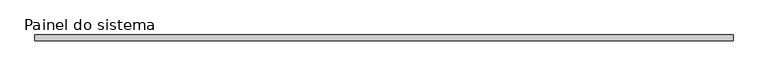
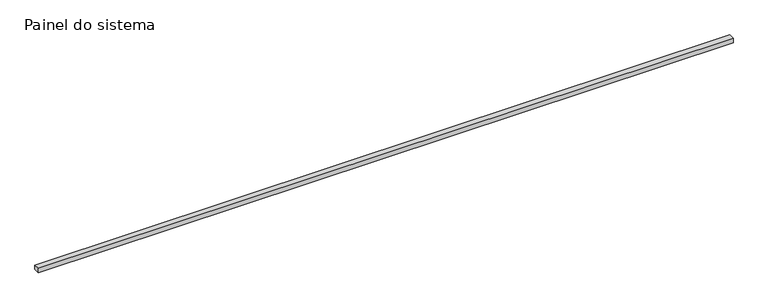
"""IFC4 building model written with IfcOpenShell, lengths in millimetres: plate geometry, Painel do sistema : Envidraçado."""

import ifcopenshell
import ifcopenshell.guid

model = None  # the IFC model being written
_history = None  # IfcOwnerHistory: only IFC2X3 demands one
_inside = {}  # id of a spatial element -> (the spatial element, [elements in it])
_under = {}  # id of a project, library or spatial element -> (it, [spatial elements below it])
_declared = {}  # id of a project -> (the project, [libraries it declares])
_typed = {}  # id of a type object -> (the type object, [elements of that type])
_made_of = {}  # id of a material, layer set ... -> (it, [elements and type objects made of it])


def new_model(schema):
    """Start an empty IFC model of exactly this schema.

    Asked for "IFC4X3", IfcOpenShell would pick the latest addendum, in which some entities
    have other attributes; the version numbers below select the first issue.
    IFC2X3 requires an IfcOwnerHistory on every rooted entity: one is made here for all.
    """
    global model, _history
    if schema == "IFC4X3":
        model = ifcopenshell.file(schema_version=(4, 3, 0, 0))
    else:
        model = ifcopenshell.file(schema=schema)
    _inside.clear()
    _under.clear()
    _declared.clear()
    _typed.clear()
    _made_of.clear()
    _history = None
    if model.schema == "IFC2X3":
        org = make("IfcOrganization", Name="unknown")
        user = make(
            "IfcPersonAndOrganization",
            ThePerson=make("IfcPerson", FamilyName="unknown"),
            TheOrganization=org,
        )
        app = make(
            "IfcApplication",
            ApplicationDeveloper=org,
            Version="unknown",
            ApplicationFullName="unknown",
            ApplicationIdentifier="unknown",
        )
        _history = make(
            "IfcOwnerHistory",
            OwningUser=user,
            OwningApplication=app,
            ChangeAction="ADDED",
            CreationDate=0,
        )
    return model


def make(cls, **values):
    """One entity of the class cls with the attributes given. An attribute that is None is left unset."""
    return model.create_entity(
        cls, **{name: value for name, value in values.items() if value is not None}
    )


def rooted(cls, **values):
    """An entity with a GlobalId (a new one), such as an element, a storey or a relation."""
    return make(cls, GlobalId=ifcopenshell.guid.new(), OwnerHistory=_history, **values)


def si_unit(unit_type, name, prefix=None):
    """IfcSIUnit, for example si_unit("LENGTHUNIT", "METRE", prefix="MILLI")."""
    return make("IfcSIUnit", UnitType=unit_type, Prefix=prefix, Name=name)


def assignment(units):
    """IfcUnitAssignment: the units of a project."""
    return None if units is None else make("IfcUnitAssignment", Units=units)


def point(xyz):
    """IfcCartesianPoint."""
    return None if xyz is None else make("IfcCartesianPoint", Coordinates=xyz)


def direction(xyz):
    """IfcDirection."""
    return None if xyz is None else make("IfcDirection", DirectionRatios=xyz)


def frame(location, z_axis=None, x_axis=None):
    """IfcAxis2Placement3D, a coordinate frame: its origin and axes. An axis left out is left unset."""
    return make(
        "IfcAxis2Placement3D",
        Location=point(location),
        Axis=direction(z_axis),
        RefDirection=direction(x_axis),
    )


def origin():
    """The frame at (0, 0, 0) with its axes left unset."""
    return frame((0.0, 0.0, 0.0))


def place(relative_to, where):
    """IfcLocalPlacement: puts the frame where relative to a parent placement (None: the world)."""
    return make(
        "IfcLocalPlacement", PlacementRelTo=relative_to, RelativePlacement=where
    )


def context(
    kind, dimensions, precision=None, world=None, true_north=None, identifier=None
):
    """IfcGeometricRepresentationContext, for example the 3D "Model" context."""
    return make(
        "IfcGeometricRepresentationContext",
        ContextIdentifier=identifier,
        ContextType=kind,
        CoordinateSpaceDimension=dimensions,
        Precision=precision,
        WorldCoordinateSystem=world,
        TrueNorth=true_north,
    )


def project(units=None, contexts=None):
    """IfcProject with its units and contexts."""
    return rooted(
        "IfcProject",
        Name="project",
        RepresentationContexts=contexts,
        UnitsInContext=assignment(units),
    )


def spatial(cls, under=None, at=None, **own):
    """A site, building, storey or space (cls), placed at a placement, below another one or the project."""
    s = rooted(cls, ObjectPlacement=at, **own)
    if under is not None:
        _under.setdefault(under.id(), (under, []))[1].append(s)
    return s


def polyline(points):
    """IfcPolyline through the points."""
    return make("IfcPolyline", Points=[point(p) for p in points])


def outline(outer, holes=None, kind="AREA"):
    """IfcArbitraryClosedProfileDef: a profile drawn as a closed curve; with holes, ...WithVoids."""
    if holes is None:
        return make("IfcArbitraryClosedProfileDef", ProfileType=kind, OuterCurve=outer)
    return make(
        "IfcArbitraryProfileDefWithVoids",
        ProfileType=kind,
        OuterCurve=outer,
        InnerCurves=holes,
    )


def extrude(swept, where, along, depth):
    """IfcExtrudedAreaSolid: the profile swept, set in the frame where, extruded along a direction by depth."""
    return make(
        "IfcExtrudedAreaSolid",
        SweptArea=swept,
        Position=where,
        ExtrudedDirection=direction(along),
        Depth=depth,
    )


def shape(context_of_items, identifier, shape_type, items):
    """IfcShapeRepresentation: the items that make up one representation, for example the "Body"."""
    return make(
        "IfcShapeRepresentation",
        ContextOfItems=context_of_items,
        RepresentationIdentifier=identifier,
        RepresentationType=shape_type,
        Items=items,
    )


def source(mapping_origin, context_of_items, identifier, shape_type, items):
    """IfcRepresentationMap: a shape defined once, which mapped items show again and again."""
    return make(
        "IfcRepresentationMap",
        MappingOrigin=mapping_origin,
        MappedRepresentation=shape(context_of_items, identifier, shape_type, items),
    )


def transform(
    local_origin,
    x_axis=None,
    y_axis=None,
    z_axis=None,
    scale=None,
    scale2=None,
    scale3=None,
    uniform=True,
):
    """IfcCartesianTransformationOperator3D, or its non-uniform kind. x_axis, y_axis, z_axis: its Axis1, 2, 3."""
    if uniform:
        return make(
            "IfcCartesianTransformationOperator3D",
            Axis1=direction(x_axis),
            Axis2=direction(y_axis),
            LocalOrigin=point(local_origin),
            Scale=scale,
            Axis3=direction(z_axis),
        )
    return make(
        "IfcCartesianTransformationOperator3DnonUniform",
        Axis1=direction(x_axis),
        Axis2=direction(y_axis),
        LocalOrigin=point(local_origin),
        Scale=scale,
        Axis3=direction(z_axis),
        Scale2=scale2,
        Scale3=scale3,
    )


def mapped(mapping_source, mapping_target):
    """IfcMappedItem: shows the shape of a source again, moved by a transform."""
    return make(
        "IfcMappedItem", MappingSource=mapping_source, MappingTarget=mapping_target
    )


def made_of(thing, what):
    """Note that an element or type object is made of a material, layer set ...; save() writes the relation."""
    if what is not None:
        _made_of.setdefault(what.id(), (what, []))[1].append(thing)
    return thing


def element(
    cls,
    number,
    at=None,
    inside=None,
    cuts=None,
    type_object=None,
    material=None,
    context=None,
    identifier="Body",
    shape_type=None,
    held_by="IfcProductDefinitionShape",
    body=None,
    shapes=None,
    **own,
):
    """One element of the class cls, such as IfcWall. Its Tag is "e" and its number.

    at: its placement. inside: the storey or other place that contains it. cuts: it is an
    opening in that element (IfcRelVoidsElement). A single representation is given by context,
    identifier, shape_type and body (its items); several are given by shapes. held_by: the class
    of the entity that holds the representations. save() writes the other relations.
    """
    e = rooted(cls, Tag="e%d" % number, ObjectPlacement=at, **own)
    if body is not None:
        shapes = [shape(context, identifier, shape_type, body)]
    if shapes is not None:
        e.Representation = make(held_by, Representations=shapes)
    if inside is not None:
        _inside.setdefault(inside.id(), (inside, []))[1].append(e)
    if cuts is not None:
        rooted(
            "IfcRelVoidsElement", RelatingBuildingElement=cuts, RelatedOpeningElement=e
        )
    if type_object is not None:
        _typed.setdefault(type_object.id(), (type_object, []))[1].append(e)
    return made_of(e, material)


def aggregate(whole, parts):
    """IfcRelAggregates: a whole, such as a stair, and the parts it consists of."""
    return rooted("IfcRelAggregates", RelatingObject=whole, RelatedObjects=parts)


def save(model, path):
    """Write the relations noted so far, then the file.

    IfcRelAggregates (storeys below a building ...), IfcRelContainedInSpatialStructure (elements
    in a storey), IfcRelDefinesByType, IfcRelAssociatesMaterial and IfcRelDeclares: one each for
    every whole, place, type object, material and project.
    """
    for whole, parts in _under.values():
        aggregate(whole, parts)
    for where, things in _inside.values():
        rooted(
            "IfcRelContainedInSpatialStructure",
            RelatedElements=things,
            RelatingStructure=where,
        )
    for kind, things in _typed.values():
        rooted("IfcRelDefinesByType", RelatedObjects=things, RelatingType=kind)
    for what, things in _made_of.values():
        rooted("IfcRelAssociatesMaterial", RelatedObjects=things, RelatingMaterial=what)
    for by, libraries in _declared.values():
        rooted("IfcRelDeclares", RelatingContext=by, RelatedDefinitions=libraries)
    model.write(path)


def painel_do_sistema_6129cf31(model_context):
    return source(origin(), model_context, "Body", "SweptSolid", [
        extrude(outline(polyline([(0.0, -1500.0), (0.0, -332.3130513), (0.0, 1500.0), (20.0931032, 1500.0), (20.0931032, -1500.0), (0.0, -1500.0)])), frame((0.0, 24.5, 0.0), z_axis=(0.0, 1.0, 0.0), x_axis=(0.0, 0.0, 1.0)), (0.0, 0.0, 1.0), 25.0),
    ])


if __name__ == "__main__":
    model = new_model("IFC4")
    model_context = context("Model", 3, world=origin())
    ifc_project = project(units=[si_unit("LENGTHUNIT", "METRE", prefix="MILLI")], contexts=[model_context])
    site = spatial("IfcSite", under=ifc_project)
    building = spatial("IfcBuilding", under=site)
    placement = place(None, origin())
    painel_do_sistema_shape = painel_do_sistema_6129cf31(model_context)
    element("IfcPlate", 1, ObjectType="Painel do sistema : Envidraçado", at=placement, inside=building, context=model_context, shape_type="MappedRepresentation", body=[
        mapped(painel_do_sistema_shape, transform((0.0, 0.0, 0.0), x_axis=(1.0, 0.0, 0.0), y_axis=(0.0, 1.0, 0.0), z_axis=(0.0, 0.0, 1.0))),
    ])
    save(model, "model.ifc")

# Revit data of these elements
# Type "Painel do sistema : Envidraçado"
#   Construction Type Id = "GSP4R"
#   Analytic Construction = "Vidraça única Pilkington 1/8 pol"
#   Visual Light Transmittance = 0.9
#   Solar Heat Gain Coefficient = 0.86
#   Heat Transfer Coefficient (U) = 6.7069 W/(m²·K)
# Element 1 (IfcPlate, "Painel do sistema : Envidraçado")
#   Materials on its faces: "Vidro"
# Materials
#   "Vidro": class "Vidro", colour RGB 0 128 192, transparency 0.9, Description = "Vidro de sílica", Cost = 0
